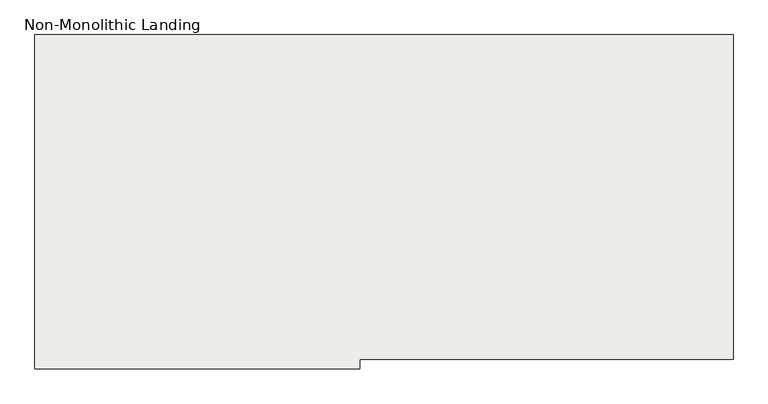
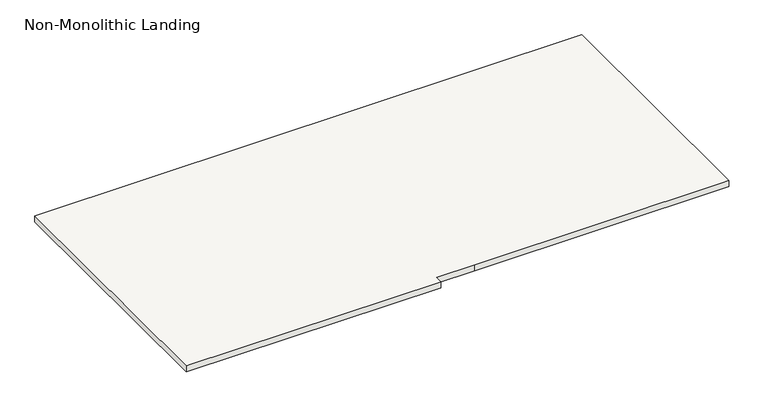
"""IFC4 building model written with IfcOpenShell, lengths in millimetres: slab geometry, Non-Monolithic Landing."""

from ifc_helpers import new_model, si_unit, frame, origin, place, context, project, spatial, polyline, outline, extrude, source, transform, mapped, element, save


def non_monolithic_landing_9d39818b(model_context):
    return source(origin(), model_context, "Body", "SweptSolid", [
        extrude(outline(polyline([(12700.0002443, 23469.9999999), (12700.0002443, 25529.9999999), (17000.0002442, 25529.9999999), (17000.0002442, 23529.9999999), (15000.0002442, 23529.9999999), (14700.0002443, 23529.9999999), (14700.0002443, 23469.9999999), (12700.0002443, 23469.9999999)])), frame((0.0, 0.0, 24950.0), z_axis=(0.0, 0.0, 1.0), x_axis=(1.0, 0.0, 0.0)), (0.0, 0.0, 1.0), 50.0),
    ])


if __name__ == "__main__":
    model = new_model("IFC4")
    model_context = context("Model", 3, world=origin())
    ifc_project = project(units=[si_unit("LENGTHUNIT", "METRE", prefix="MILLI")], contexts=[model_context])
    site = spatial("IfcSite", under=ifc_project)
    building = spatial("IfcBuilding", under=site)
    placement = place(None, origin())
    non_monolithic_landing_shape = non_monolithic_landing_9d39818b(model_context)
    element("IfcSlab", 1, ObjectType="Non-Monolithic Landing", at=placement, inside=building, context=model_context, shape_type="MappedRepresentation", body=[
        mapped(non_monolithic_landing_shape, transform((0.0, 0.0, 0.0), x_axis=(1.0, 0.0, 0.0), y_axis=(0.0, 1.0, 0.0), z_axis=(0.0, 0.0, 1.0))),
    ])
    save(model, "model.ifc")
